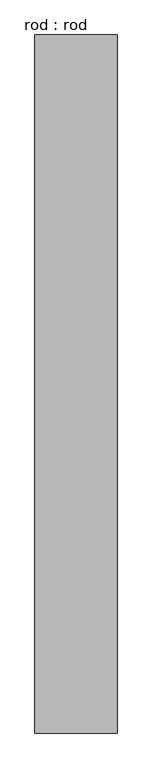
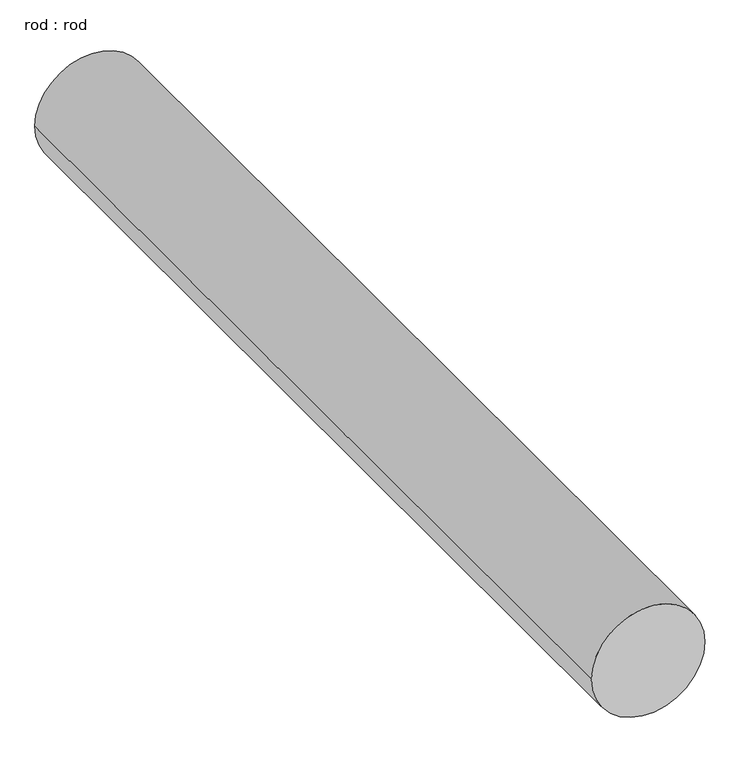
"""IFC4 building model written with IfcOpenShell, lengths in millimetres: proxy geometry, rod : rod."""

from ifc_helpers import new_model, si_unit, point, frame, frame_2d, origin, place, context, project, spatial, circle_curve, trimmed, segment, composite_curve, outline, extrude, source, transform, mapped, element, save


def rod_rod_368149a3(model_context):
    return source(origin(), model_context, "Body", "SweptSolid", [
        extrude(outline(composite_curve([segment(trimmed(circle_curve(frame_2d((0.0108462, 0.0)), 200.0), [point((0.0108462, 200.0))], [point((0.0108462, -200.0))], False, "CARTESIAN"), True, "CONTINUOUS"), segment(trimmed(circle_curve(frame_2d((0.0108462, 0.0)), 200.0), [point((0.0108462, -200.0))], [point((0.0108462, 200.0))], False, "CARTESIAN"), True, "CONTINUOUS")], self_intersect=False)), frame((0.0, 2392.7286153, 0.0), z_axis=(0.0, 1.0, 0.0), x_axis=(0.0, 0.0, 1.0)), (0.0, 0.0, 1.0), 3400.0),
    ])


if __name__ == "__main__":
    model = new_model("IFC4")
    model_context = context("Model", 3, world=origin())
    ifc_project = project(units=[si_unit("LENGTHUNIT", "METRE", prefix="MILLI")], contexts=[model_context])
    site = spatial("IfcSite", under=ifc_project)
    building = spatial("IfcBuilding", under=site)
    placement = place(None, origin())
    rod_rod_shape = rod_rod_368149a3(model_context)
    element("IfcBuildingElementProxy", 1, Name="rod : rod", ObjectType="rod : rod", at=placement, inside=building, context=model_context, shape_type="MappedRepresentation", body=[
        mapped(rod_rod_shape, transform((0.0, 0.0, 0.0), x_axis=(1.0, 0.0, 0.0), y_axis=(0.0, 1.0, 0.0), z_axis=(0.0, 0.0, 1.0))),
    ])
    save(model, "model.ifc")

# Revit data of these elements
# Type "rod : rod"
#   Default Elevation = 0
